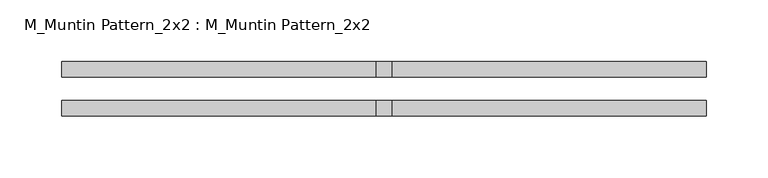
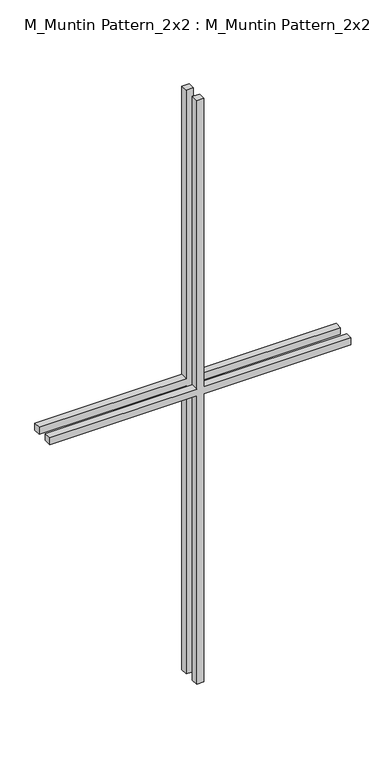
"""IFC4 building model written with IfcOpenShell, lengths in millimetres: proxy geometry, M_Muntin Pattern_2x2 : M_Muntin Pattern_2x2."""

from ifc_helpers import new_model, si_unit, frame, origin, place, context, project, spatial, polyline, outline, extrude, source, transform, mapped, element, save


def m_muntin_pattern_2x2_m_muntin_pattern_2x2_c2d27229(model_context):
    return source(origin(), model_context, "Body", "SweptSolid", [
        extrude(outline(polyline([(542.925, -6.35), (542.925, -261.9375), (530.225, -261.9375), (530.225, -6.35), (0.0, -6.35), (0.0, 6.35), (530.225, 6.35), (530.225, 261.9375), (542.925, 261.9375), (542.925, 6.35), (1073.15, 6.35), (1073.15, -6.35), (542.925, -6.35)])), frame((0.0, -22.225, 0.0), z_axis=(0.0, 1.0, 0.0), x_axis=(0.0, 0.0, 1.0)), (0.0, 0.0, 1.0), 12.7),
        extrude(outline(polyline([(542.925, -6.35), (542.925, -261.9375), (530.225, -261.9375), (530.225, -6.35), (0.0, -6.35), (0.0, 6.35), (530.225, 6.35), (530.225, 261.9375), (542.925, 261.9375), (542.925, 6.35), (1073.15, 6.35), (1073.15, -6.35), (542.925, -6.35)])), frame((0.0, 9.525, 0.0), z_axis=(0.0, 1.0, 0.0), x_axis=(0.0, 0.0, 1.0)), (0.0, 0.0, 1.0), 12.7),
    ])


if __name__ == "__main__":
    model = new_model("IFC4")
    model_context = context("Model", 3, world=origin())
    ifc_project = project(units=[si_unit("LENGTHUNIT", "METRE", prefix="MILLI")], contexts=[model_context])
    site = spatial("IfcSite", under=ifc_project)
    building = spatial("IfcBuilding", under=site)
    placement = place(None, origin())
    m_muntin_pattern_2x2_m_muntin_pattern_2x2_shape = m_muntin_pattern_2x2_m_muntin_pattern_2x2_c2d27229(model_context)
    element("IfcBuildingElementProxy", 1, Name="M_Muntin Pattern_2x2 : M_Muntin Pattern_2x2", ObjectType="M_Muntin Pattern_2x2 : M_Muntin Pattern_2x2", at=placement, inside=building, context=model_context, shape_type="MappedRepresentation", body=[
        mapped(m_muntin_pattern_2x2_m_muntin_pattern_2x2_shape, transform((0.0, 0.0, 0.0), x_axis=(1.0, 0.0, 0.0), y_axis=(0.0, 1.0, 0.0), z_axis=(0.0, 0.0, 1.0))),
    ])
    save(model, "model.ifc")

# Revit data of these elements
# Type "M_Muntin Pattern_2x2 : M_Muntin Pattern_2x2"
#   Width [instance default] = 3' - 11.24409"
#   Thickness = 0' - 0 1/2"
#   Height [instance default] = 3' - 11.24409"
#   Distance = 0' - 0 3/4"
#   Interior Material [instance default] = none
#   Exterior Material [instance default] = none
#   Default Elevation = 0
# Element 1 (IfcBuildingElementProxy, "M_Muntin Pattern_2x2 : M_Muntin Pattern_2x2")
#   Width = 1' - 8 5/8"
#   Height = 3' - 6 1/4"
#   Interior Material = Wood - Stained
#   Exterior Material = Clad - White
#   Materials on its faces: "Clad - White", "Wood - Stained"
# Materials
#   "Clad - White": class "Wood", colour RGB 242 242 238, transparency 0, Cost = 0
#   "Wood - Stained": class "Wood", colour RGB 224 178 126, transparency 0, Cost = 0
